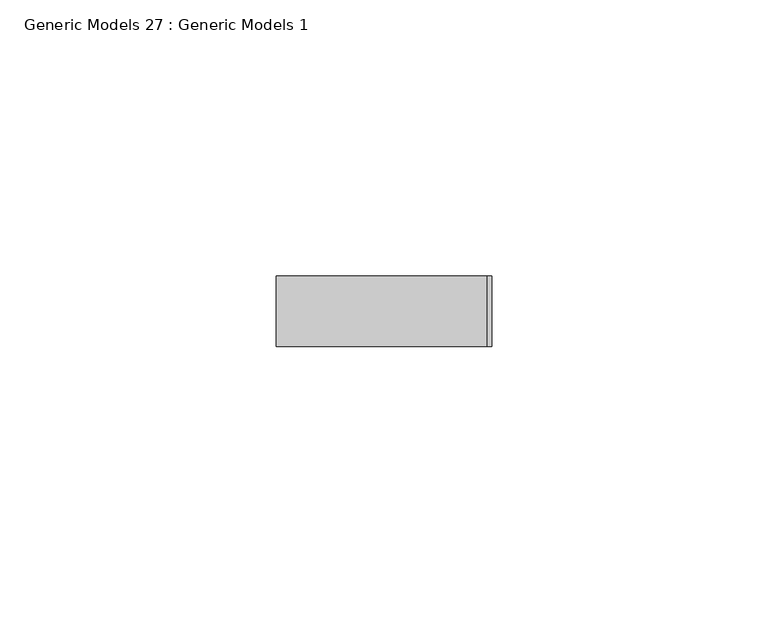
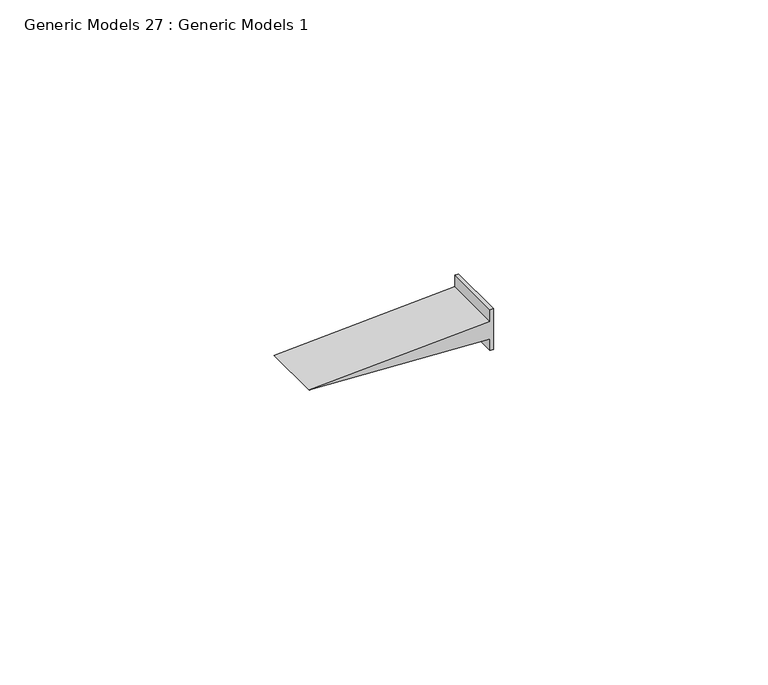
"""IFC4 building model written with IfcOpenShell, lengths in millimetres: proxy geometry, Generic Models 27 : Generic Models 1."""

import ifcopenshell
import ifcopenshell.guid

model = None  # the IFC model being written
_history = None  # IfcOwnerHistory: only IFC2X3 demands one
_inside = {}  # id of a spatial element -> (the spatial element, [elements in it])
_under = {}  # id of a project, library or spatial element -> (it, [spatial elements below it])
_declared = {}  # id of a project -> (the project, [libraries it declares])
_typed = {}  # id of a type object -> (the type object, [elements of that type])
_made_of = {}  # id of a material, layer set ... -> (it, [elements and type objects made of it])


def new_model(schema):
    """Start an empty IFC model of exactly this schema.

    Asked for "IFC4X3", IfcOpenShell would pick the latest addendum, in which some entities
    have other attributes; the version numbers below select the first issue.
    IFC2X3 requires an IfcOwnerHistory on every rooted entity: one is made here for all.
    """
    global model, _history
    if schema == "IFC4X3":
        model = ifcopenshell.file(schema_version=(4, 3, 0, 0))
    else:
        model = ifcopenshell.file(schema=schema)
    _inside.clear()
    _under.clear()
    _declared.clear()
    _typed.clear()
    _made_of.clear()
    _history = None
    if model.schema == "IFC2X3":
        org = make("IfcOrganization", Name="unknown")
        user = make(
            "IfcPersonAndOrganization",
            ThePerson=make("IfcPerson", FamilyName="unknown"),
            TheOrganization=org,
        )
        app = make(
            "IfcApplication",
            ApplicationDeveloper=org,
            Version="unknown",
            ApplicationFullName="unknown",
            ApplicationIdentifier="unknown",
        )
        _history = make(
            "IfcOwnerHistory",
            OwningUser=user,
            OwningApplication=app,
            ChangeAction="ADDED",
            CreationDate=0,
        )
    return model


def make(cls, **values):
    """One entity of the class cls with the attributes given. An attribute that is None is left unset."""
    return model.create_entity(
        cls, **{name: value for name, value in values.items() if value is not None}
    )


def rooted(cls, **values):
    """An entity with a GlobalId (a new one), such as an element, a storey or a relation."""
    return make(cls, GlobalId=ifcopenshell.guid.new(), OwnerHistory=_history, **values)


def si_unit(unit_type, name, prefix=None):
    """IfcSIUnit, for example si_unit("LENGTHUNIT", "METRE", prefix="MILLI")."""
    return make("IfcSIUnit", UnitType=unit_type, Prefix=prefix, Name=name)


def assignment(units):
    """IfcUnitAssignment: the units of a project."""
    return None if units is None else make("IfcUnitAssignment", Units=units)


def point(xyz):
    """IfcCartesianPoint."""
    return None if xyz is None else make("IfcCartesianPoint", Coordinates=xyz)


def direction(xyz):
    """IfcDirection."""
    return None if xyz is None else make("IfcDirection", DirectionRatios=xyz)


def frame(location, z_axis=None, x_axis=None):
    """IfcAxis2Placement3D, a coordinate frame: its origin and axes. An axis left out is left unset."""
    return make(
        "IfcAxis2Placement3D",
        Location=point(location),
        Axis=direction(z_axis),
        RefDirection=direction(x_axis),
    )


def origin():
    """The frame at (0, 0, 0) with its axes left unset."""
    return frame((0.0, 0.0, 0.0))


def place(relative_to, where):
    """IfcLocalPlacement: puts the frame where relative to a parent placement (None: the world)."""
    return make(
        "IfcLocalPlacement", PlacementRelTo=relative_to, RelativePlacement=where
    )


def context(
    kind, dimensions, precision=None, world=None, true_north=None, identifier=None
):
    """IfcGeometricRepresentationContext, for example the 3D "Model" context."""
    return make(
        "IfcGeometricRepresentationContext",
        ContextIdentifier=identifier,
        ContextType=kind,
        CoordinateSpaceDimension=dimensions,
        Precision=precision,
        WorldCoordinateSystem=world,
        TrueNorth=true_north,
    )


def project(units=None, contexts=None):
    """IfcProject with its units and contexts."""
    return rooted(
        "IfcProject",
        Name="project",
        RepresentationContexts=contexts,
        UnitsInContext=assignment(units),
    )


def spatial(cls, under=None, at=None, **own):
    """A site, building, storey or space (cls), placed at a placement, below another one or the project."""
    s = rooted(cls, ObjectPlacement=at, **own)
    if under is not None:
        _under.setdefault(under.id(), (under, []))[1].append(s)
    return s


def polyline(points):
    """IfcPolyline through the points."""
    return make("IfcPolyline", Points=[point(p) for p in points])


def outline(outer, holes=None, kind="AREA"):
    """IfcArbitraryClosedProfileDef: a profile drawn as a closed curve; with holes, ...WithVoids."""
    if holes is None:
        return make("IfcArbitraryClosedProfileDef", ProfileType=kind, OuterCurve=outer)
    return make(
        "IfcArbitraryProfileDefWithVoids",
        ProfileType=kind,
        OuterCurve=outer,
        InnerCurves=holes,
    )


def extrude(swept, where, along, depth):
    """IfcExtrudedAreaSolid: the profile swept, set in the frame where, extruded along a direction by depth."""
    return make(
        "IfcExtrudedAreaSolid",
        SweptArea=swept,
        Position=where,
        ExtrudedDirection=direction(along),
        Depth=depth,
    )


def shape(context_of_items, identifier, shape_type, items):
    """IfcShapeRepresentation: the items that make up one representation, for example the "Body"."""
    return make(
        "IfcShapeRepresentation",
        ContextOfItems=context_of_items,
        RepresentationIdentifier=identifier,
        RepresentationType=shape_type,
        Items=items,
    )


def source(mapping_origin, context_of_items, identifier, shape_type, items):
    """IfcRepresentationMap: a shape defined once, which mapped items show again and again."""
    return make(
        "IfcRepresentationMap",
        MappingOrigin=mapping_origin,
        MappedRepresentation=shape(context_of_items, identifier, shape_type, items),
    )


def transform(
    local_origin,
    x_axis=None,
    y_axis=None,
    z_axis=None,
    scale=None,
    scale2=None,
    scale3=None,
    uniform=True,
):
    """IfcCartesianTransformationOperator3D, or its non-uniform kind. x_axis, y_axis, z_axis: its Axis1, 2, 3."""
    if uniform:
        return make(
            "IfcCartesianTransformationOperator3D",
            Axis1=direction(x_axis),
            Axis2=direction(y_axis),
            LocalOrigin=point(local_origin),
            Scale=scale,
            Axis3=direction(z_axis),
        )
    return make(
        "IfcCartesianTransformationOperator3DnonUniform",
        Axis1=direction(x_axis),
        Axis2=direction(y_axis),
        LocalOrigin=point(local_origin),
        Scale=scale,
        Axis3=direction(z_axis),
        Scale2=scale2,
        Scale3=scale3,
    )


def mapped(mapping_source, mapping_target):
    """IfcMappedItem: shows the shape of a source again, moved by a transform."""
    return make(
        "IfcMappedItem", MappingSource=mapping_source, MappingTarget=mapping_target
    )


def made_of(thing, what):
    """Note that an element or type object is made of a material, layer set ...; save() writes the relation."""
    if what is not None:
        _made_of.setdefault(what.id(), (what, []))[1].append(thing)
    return thing


def element(
    cls,
    number,
    at=None,
    inside=None,
    cuts=None,
    type_object=None,
    material=None,
    context=None,
    identifier="Body",
    shape_type=None,
    held_by="IfcProductDefinitionShape",
    body=None,
    shapes=None,
    **own,
):
    """One element of the class cls, such as IfcWall. Its Tag is "e" and its number.

    at: its placement. inside: the storey or other place that contains it. cuts: it is an
    opening in that element (IfcRelVoidsElement). A single representation is given by context,
    identifier, shape_type and body (its items); several are given by shapes. held_by: the class
    of the entity that holds the representations. save() writes the other relations.
    """
    e = rooted(cls, Tag="e%d" % number, ObjectPlacement=at, **own)
    if body is not None:
        shapes = [shape(context, identifier, shape_type, body)]
    if shapes is not None:
        e.Representation = make(held_by, Representations=shapes)
    if inside is not None:
        _inside.setdefault(inside.id(), (inside, []))[1].append(e)
    if cuts is not None:
        rooted(
            "IfcRelVoidsElement", RelatingBuildingElement=cuts, RelatedOpeningElement=e
        )
    if type_object is not None:
        _typed.setdefault(type_object.id(), (type_object, []))[1].append(e)
    return made_of(e, material)


def aggregate(whole, parts):
    """IfcRelAggregates: a whole, such as a stair, and the parts it consists of."""
    return rooted("IfcRelAggregates", RelatingObject=whole, RelatedObjects=parts)


def save(model, path):
    """Write the relations noted so far, then the file.

    IfcRelAggregates (storeys below a building ...), IfcRelContainedInSpatialStructure (elements
    in a storey), IfcRelDefinesByType, IfcRelAssociatesMaterial and IfcRelDeclares: one each for
    every whole, place, type object, material and project.
    """
    for whole, parts in _under.values():
        aggregate(whole, parts)
    for where, things in _inside.values():
        rooted(
            "IfcRelContainedInSpatialStructure",
            RelatedElements=things,
            RelatingStructure=where,
        )
    for kind, things in _typed.values():
        rooted("IfcRelDefinesByType", RelatedObjects=things, RelatingType=kind)
    for what, things in _made_of.values():
        rooted("IfcRelAssociatesMaterial", RelatedObjects=things, RelatingMaterial=what)
    for by, libraries in _declared.values():
        rooted("IfcRelDeclares", RelatingContext=by, RelatedDefinitions=libraries)
    model.write(path)


def generic_models_27_generic_models_1_58db4025(model_context):
    return source(origin(), model_context, "Body", "SweptSolid", [
        extrude(outline(polyline([(2414.3721662, 49800.66875), (2414.3721662, 49799.875), (2411.8223026, 49799.875), (2409.8255662, 49761.775), (2407.8288298, 49799.875), (2405.2789662, 49799.875), (2405.2789662, 49800.66875), (2414.3721662, 49800.66875)])), frame((0.0, 565.15, 0.0), z_axis=(0.0, 1.0, 0.0), x_axis=(0.0, 0.0, 1.0)), (0.0, 0.0, 1.0), 12.7),
    ])


if __name__ == "__main__":
    model = new_model("IFC4")
    model_context = context("Model", 3, world=origin())
    ifc_project = project(units=[si_unit("LENGTHUNIT", "METRE", prefix="MILLI")], contexts=[model_context])
    site = spatial("IfcSite", under=ifc_project)
    building = spatial("IfcBuilding", under=site)
    placement = place(None, origin())
    generic_models_27_generic_models_1_shape = generic_models_27_generic_models_1_58db4025(model_context)
    element("IfcBuildingElementProxy", 1, Name="Generic Models 27 : Generic Models 1", ObjectType="Generic Models 27 : Generic Models 1", at=placement, inside=building, context=model_context, shape_type="MappedRepresentation", body=[
        mapped(generic_models_27_generic_models_1_shape, transform((0.0, 0.0, 0.0), x_axis=(1.0, 0.0, 0.0), y_axis=(0.0, 1.0, 0.0), z_axis=(0.0, 0.0, 1.0))),
    ])
    save(model, "model.ifc")

# Revit data of these elements
# Element 1 (IfcBuildingElementProxy, "Generic Models 27 : Generic Models 1")
#   Materials on its faces: "ATTACH GYPSUM BOARD TO STUDS AND NOT TO TOP TRACK"
# Materials
#   "ATTACH GYPSUM BOARD TO STUDS AND NOT TO TOP TRACK": class "Generic", colour RGB 48 48 48, transparency 0, Cost = 0
